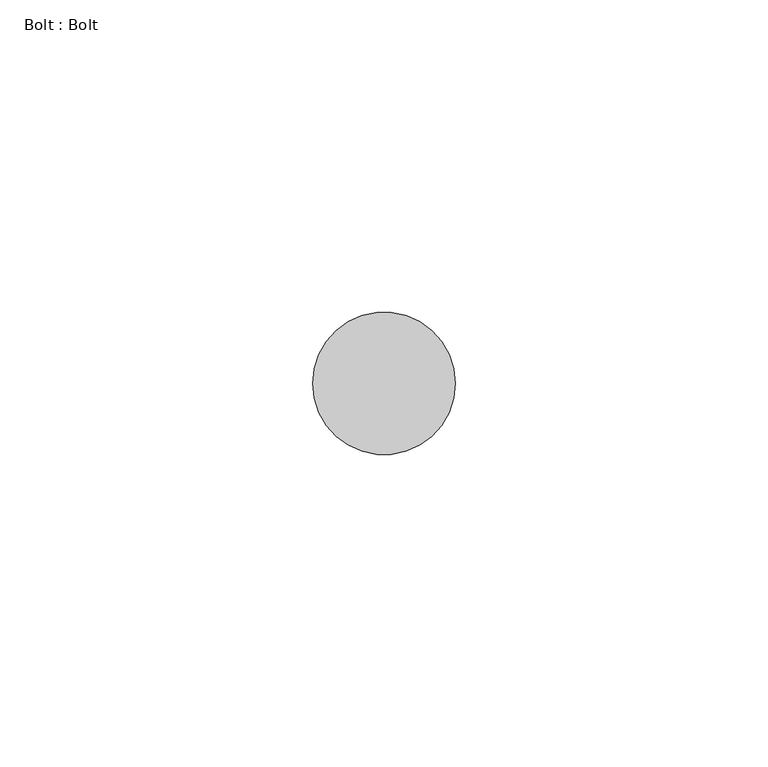
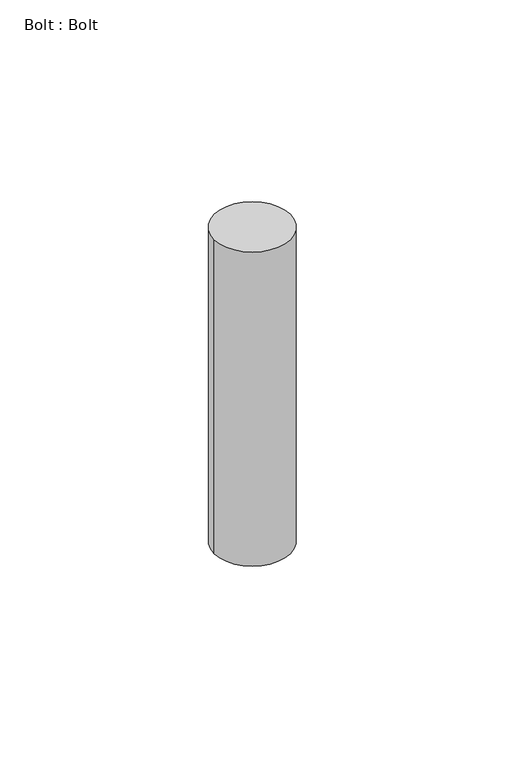
"""IFC4 building model written with IfcOpenShell, lengths in millimetres: proxy geometry, Bolt : Bolt."""

import ifcopenshell
import ifcopenshell.guid

model = None  # the IFC model being written
_history = None  # IfcOwnerHistory: only IFC2X3 demands one
_inside = {}  # id of a spatial element -> (the spatial element, [elements in it])
_under = {}  # id of a project, library or spatial element -> (it, [spatial elements below it])
_declared = {}  # id of a project -> (the project, [libraries it declares])
_typed = {}  # id of a type object -> (the type object, [elements of that type])
_made_of = {}  # id of a material, layer set ... -> (it, [elements and type objects made of it])


def new_model(schema):
    """Start an empty IFC model of exactly this schema.

    Asked for "IFC4X3", IfcOpenShell would pick the latest addendum, in which some entities
    have other attributes; the version numbers below select the first issue.
    IFC2X3 requires an IfcOwnerHistory on every rooted entity: one is made here for all.
    """
    global model, _history
    if schema == "IFC4X3":
        model = ifcopenshell.file(schema_version=(4, 3, 0, 0))
    else:
        model = ifcopenshell.file(schema=schema)
    _inside.clear()
    _under.clear()
    _declared.clear()
    _typed.clear()
    _made_of.clear()
    _history = None
    if model.schema == "IFC2X3":
        org = make("IfcOrganization", Name="unknown")
        user = make(
            "IfcPersonAndOrganization",
            ThePerson=make("IfcPerson", FamilyName="unknown"),
            TheOrganization=org,
        )
        app = make(
            "IfcApplication",
            ApplicationDeveloper=org,
            Version="unknown",
            ApplicationFullName="unknown",
            ApplicationIdentifier="unknown",
        )
        _history = make(
            "IfcOwnerHistory",
            OwningUser=user,
            OwningApplication=app,
            ChangeAction="ADDED",
            CreationDate=0,
        )
    return model


def make(cls, **values):
    """One entity of the class cls with the attributes given. An attribute that is None is left unset."""
    return model.create_entity(
        cls, **{name: value for name, value in values.items() if value is not None}
    )


def rooted(cls, **values):
    """An entity with a GlobalId (a new one), such as an element, a storey or a relation."""
    return make(cls, GlobalId=ifcopenshell.guid.new(), OwnerHistory=_history, **values)


def si_unit(unit_type, name, prefix=None):
    """IfcSIUnit, for example si_unit("LENGTHUNIT", "METRE", prefix="MILLI")."""
    return make("IfcSIUnit", UnitType=unit_type, Prefix=prefix, Name=name)


def assignment(units):
    """IfcUnitAssignment: the units of a project."""
    return None if units is None else make("IfcUnitAssignment", Units=units)


def point(xyz):
    """IfcCartesianPoint."""
    return None if xyz is None else make("IfcCartesianPoint", Coordinates=xyz)


def direction(xyz):
    """IfcDirection."""
    return None if xyz is None else make("IfcDirection", DirectionRatios=xyz)


def frame(location, z_axis=None, x_axis=None):
    """IfcAxis2Placement3D, a coordinate frame: its origin and axes. An axis left out is left unset."""
    return make(
        "IfcAxis2Placement3D",
        Location=point(location),
        Axis=direction(z_axis),
        RefDirection=direction(x_axis),
    )


def frame_2d(location, x_axis=None):
    """IfcAxis2Placement2D, a coordinate frame in the plane: its origin and x axis."""
    return make(
        "IfcAxis2Placement2D", Location=point(location), RefDirection=direction(x_axis)
    )


def origin():
    """The frame at (0, 0, 0) with its axes left unset."""
    return frame((0.0, 0.0, 0.0))


def place(relative_to, where):
    """IfcLocalPlacement: puts the frame where relative to a parent placement (None: the world)."""
    return make(
        "IfcLocalPlacement", PlacementRelTo=relative_to, RelativePlacement=where
    )


def context(
    kind, dimensions, precision=None, world=None, true_north=None, identifier=None
):
    """IfcGeometricRepresentationContext, for example the 3D "Model" context."""
    return make(
        "IfcGeometricRepresentationContext",
        ContextIdentifier=identifier,
        ContextType=kind,
        CoordinateSpaceDimension=dimensions,
        Precision=precision,
        WorldCoordinateSystem=world,
        TrueNorth=true_north,
    )


def project(units=None, contexts=None):
    """IfcProject with its units and contexts."""
    return rooted(
        "IfcProject",
        Name="project",
        RepresentationContexts=contexts,
        UnitsInContext=assignment(units),
    )


def spatial(cls, under=None, at=None, **own):
    """A site, building, storey or space (cls), placed at a placement, below another one or the project."""
    s = rooted(cls, ObjectPlacement=at, **own)
    if under is not None:
        _under.setdefault(under.id(), (under, []))[1].append(s)
    return s


def circle_curve(where, radius):
    """IfcCircle in the frame where."""
    return make("IfcCircle", Position=where, Radius=radius)


def trimmed(basis, trim1, trim2, sense, master):
    """IfcTrimmedCurve: the piece of a basis curve between two trims."""
    return make(
        "IfcTrimmedCurve",
        BasisCurve=basis,
        Trim1=trim1,
        Trim2=trim2,
        SenseAgreement=sense,
        MasterRepresentation=master,
    )


def segment(curve, same_sense, transition):
    """IfcCompositeCurveSegment."""
    return make(
        "IfcCompositeCurveSegment",
        Transition=transition,
        SameSense=same_sense,
        ParentCurve=curve,
    )


def composite_curve(segments, self_intersect=None):
    """IfcCompositeCurve: segments joined end to end."""
    return make("IfcCompositeCurve", Segments=segments, SelfIntersect=self_intersect)


def outline(outer, holes=None, kind="AREA"):
    """IfcArbitraryClosedProfileDef: a profile drawn as a closed curve; with holes, ...WithVoids."""
    if holes is None:
        return make("IfcArbitraryClosedProfileDef", ProfileType=kind, OuterCurve=outer)
    return make(
        "IfcArbitraryProfileDefWithVoids",
        ProfileType=kind,
        OuterCurve=outer,
        InnerCurves=holes,
    )


def extrude(swept, where, along, depth):
    """IfcExtrudedAreaSolid: the profile swept, set in the frame where, extruded along a direction by depth."""
    return make(
        "IfcExtrudedAreaSolid",
        SweptArea=swept,
        Position=where,
        ExtrudedDirection=direction(along),
        Depth=depth,
    )


def shape(context_of_items, identifier, shape_type, items):
    """IfcShapeRepresentation: the items that make up one representation, for example the "Body"."""
    return make(
        "IfcShapeRepresentation",
        ContextOfItems=context_of_items,
        RepresentationIdentifier=identifier,
        RepresentationType=shape_type,
        Items=items,
    )


def source(mapping_origin, context_of_items, identifier, shape_type, items):
    """IfcRepresentationMap: a shape defined once, which mapped items show again and again."""
    return make(
        "IfcRepresentationMap",
        MappingOrigin=mapping_origin,
        MappedRepresentation=shape(context_of_items, identifier, shape_type, items),
    )


def transform(
    local_origin,
    x_axis=None,
    y_axis=None,
    z_axis=None,
    scale=None,
    scale2=None,
    scale3=None,
    uniform=True,
):
    """IfcCartesianTransformationOperator3D, or its non-uniform kind. x_axis, y_axis, z_axis: its Axis1, 2, 3."""
    if uniform:
        return make(
            "IfcCartesianTransformationOperator3D",
            Axis1=direction(x_axis),
            Axis2=direction(y_axis),
            LocalOrigin=point(local_origin),
            Scale=scale,
            Axis3=direction(z_axis),
        )
    return make(
        "IfcCartesianTransformationOperator3DnonUniform",
        Axis1=direction(x_axis),
        Axis2=direction(y_axis),
        LocalOrigin=point(local_origin),
        Scale=scale,
        Axis3=direction(z_axis),
        Scale2=scale2,
        Scale3=scale3,
    )


def mapped(mapping_source, mapping_target):
    """IfcMappedItem: shows the shape of a source again, moved by a transform."""
    return make(
        "IfcMappedItem", MappingSource=mapping_source, MappingTarget=mapping_target
    )


def made_of(thing, what):
    """Note that an element or type object is made of a material, layer set ...; save() writes the relation."""
    if what is not None:
        _made_of.setdefault(what.id(), (what, []))[1].append(thing)
    return thing


def element(
    cls,
    number,
    at=None,
    inside=None,
    cuts=None,
    type_object=None,
    material=None,
    context=None,
    identifier="Body",
    shape_type=None,
    held_by="IfcProductDefinitionShape",
    body=None,
    shapes=None,
    **own,
):
    """One element of the class cls, such as IfcWall. Its Tag is "e" and its number.

    at: its placement. inside: the storey or other place that contains it. cuts: it is an
    opening in that element (IfcRelVoidsElement). A single representation is given by context,
    identifier, shape_type and body (its items); several are given by shapes. held_by: the class
    of the entity that holds the representations. save() writes the other relations.
    """
    e = rooted(cls, Tag="e%d" % number, ObjectPlacement=at, **own)
    if body is not None:
        shapes = [shape(context, identifier, shape_type, body)]
    if shapes is not None:
        e.Representation = make(held_by, Representations=shapes)
    if inside is not None:
        _inside.setdefault(inside.id(), (inside, []))[1].append(e)
    if cuts is not None:
        rooted(
            "IfcRelVoidsElement", RelatingBuildingElement=cuts, RelatedOpeningElement=e
        )
    if type_object is not None:
        _typed.setdefault(type_object.id(), (type_object, []))[1].append(e)
    return made_of(e, material)


def aggregate(whole, parts):
    """IfcRelAggregates: a whole, such as a stair, and the parts it consists of."""
    return rooted("IfcRelAggregates", RelatingObject=whole, RelatedObjects=parts)


def save(model, path):
    """Write the relations noted so far, then the file.

    IfcRelAggregates (storeys below a building ...), IfcRelContainedInSpatialStructure (elements
    in a storey), IfcRelDefinesByType, IfcRelAssociatesMaterial and IfcRelDeclares: one each for
    every whole, place, type object, material and project.
    """
    for whole, parts in _under.values():
        aggregate(whole, parts)
    for where, things in _inside.values():
        rooted(
            "IfcRelContainedInSpatialStructure",
            RelatedElements=things,
            RelatingStructure=where,
        )
    for kind, things in _typed.values():
        rooted("IfcRelDefinesByType", RelatedObjects=things, RelatingType=kind)
    for what, things in _made_of.values():
        rooted("IfcRelAssociatesMaterial", RelatedObjects=things, RelatingMaterial=what)
    for by, libraries in _declared.values():
        rooted("IfcRelDeclares", RelatingContext=by, RelatedDefinitions=libraries)
    model.write(path)


def bolt_bolt_d23a2250(model_context):
    return source(origin(), model_context, "Body", "SweptSolid", [
        extrude(outline(composite_curve([segment(trimmed(circle_curve(frame_2d((7251.9702148, -1781.8449707)), 11.4045168), [point((7240.565698, -1781.8449707))], [point((7263.3747317, -1781.8449707))], False, "CARTESIAN"), True, "CONTINUOUS"), segment(trimmed(circle_curve(frame_2d((7251.9702148, -1781.8449707)), 11.4045168), [point((7263.3747317, -1781.8449707))], [point((7240.565698, -1781.8449707))], False, "CARTESIAN"), True, "CONTINUOUS")], self_intersect=False)), frame((0.0, 0.0, 39994.0914664), z_axis=(0.0, 0.0, 1.0), x_axis=(1.0, 0.0, 0.0)), (0.0, 0.0, 1.0), 99.5545336),
    ])


if __name__ == "__main__":
    model = new_model("IFC4")
    model_context = context("Model", 3, world=origin())
    ifc_project = project(units=[si_unit("LENGTHUNIT", "METRE", prefix="MILLI")], contexts=[model_context])
    site = spatial("IfcSite", under=ifc_project)
    building = spatial("IfcBuilding", under=site)
    placement = place(None, origin())
    bolt_bolt_shape = bolt_bolt_d23a2250(model_context)
    element("IfcBuildingElementProxy", 1, Name="Bolt : Bolt", ObjectType="Bolt : Bolt", at=placement, inside=building, context=model_context, shape_type="MappedRepresentation", body=[
        mapped(bolt_bolt_shape, transform((0.0, 0.0, 0.0), x_axis=(1.0, 0.0, 0.0), y_axis=(0.0, 1.0, 0.0), z_axis=(0.0, 0.0, 1.0))),
    ])
    save(model, "model.ifc")

# Revit data of these elements
# Type "Bolt : Bolt"
#   NameOverride = "Bolt"
# Element 1 (IfcBuildingElementProxy, "Bolt : Bolt")
#   Materials on its faces: "BOLTS CONCEALED BY FLOOR FINISH"
# Materials
#   "BOLTS CONCEALED BY FLOOR FINISH": class "Unassigned", colour RGB 128 128 128, transparency 0
